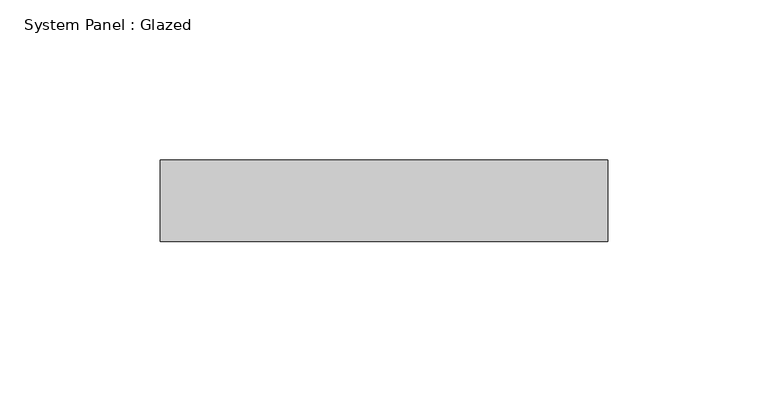
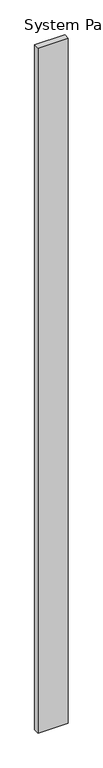
"""IFC4 building model written with IfcOpenShell, lengths in millimetres: plate geometry, System Panel : Glazed."""

from ifc_helpers import new_model, si_unit, origin, origin_with_axes, place, context, project, spatial, polyline, outline, extrude, source, transform, mapped, element, save


def system_panel_glazed_bf13c76d(model_context):
    return source(origin(), model_context, "Body", "SweptSolid", [
        extrude(outline(polyline([(69.649919, 19.05), (-69.649919, 19.05), (-69.649919, 44.45), (69.649919, 44.45), (69.649919, 19.05)])), origin_with_axes(), (0.0, 0.0, 1.0), 3352.8),
    ])


if __name__ == "__main__":
    model = new_model("IFC4")
    model_context = context("Model", 3, world=origin())
    ifc_project = project(units=[si_unit("LENGTHUNIT", "METRE", prefix="MILLI")], contexts=[model_context])
    site = spatial("IfcSite", under=ifc_project)
    building = spatial("IfcBuilding", under=site)
    placement = place(None, origin())
    system_panel_glazed_shape = system_panel_glazed_bf13c76d(model_context)
    element("IfcPlate", 1, ObjectType="System Panel : Glazed", at=placement, inside=building, context=model_context, shape_type="MappedRepresentation", body=[
        mapped(system_panel_glazed_shape, transform((0.0, 0.0, 0.0), x_axis=(1.0, 0.0, 0.0), y_axis=(0.0, 1.0, 0.0), z_axis=(0.0, 0.0, 1.0))),
    ])
    save(model, "model.ifc")

# Revit data of these elements
# Type "System Panel : Glazed"
#   Construction Type Id = "GSP4R"
#   Analytic Construction = "1/8 in Pilkington single glazing"
#   Visual Light Transmittance = 0.9
#   Solar Heat Gain Coefficient = 0.86
#   Heat Transfer Coefficient (U) = 1.18115 BTU/(h·ft²·°F)
#   Define Thermal Properties by = 1
# Element 1 (IfcPlate, "System Panel : Glazed")
#   Materials on its faces: "Glass"
# Materials
#   "Glass": class "Glass", colour RGB 0 128 192, transparency 0.75, Description = "Soda Lime Glass", Cost = 0
